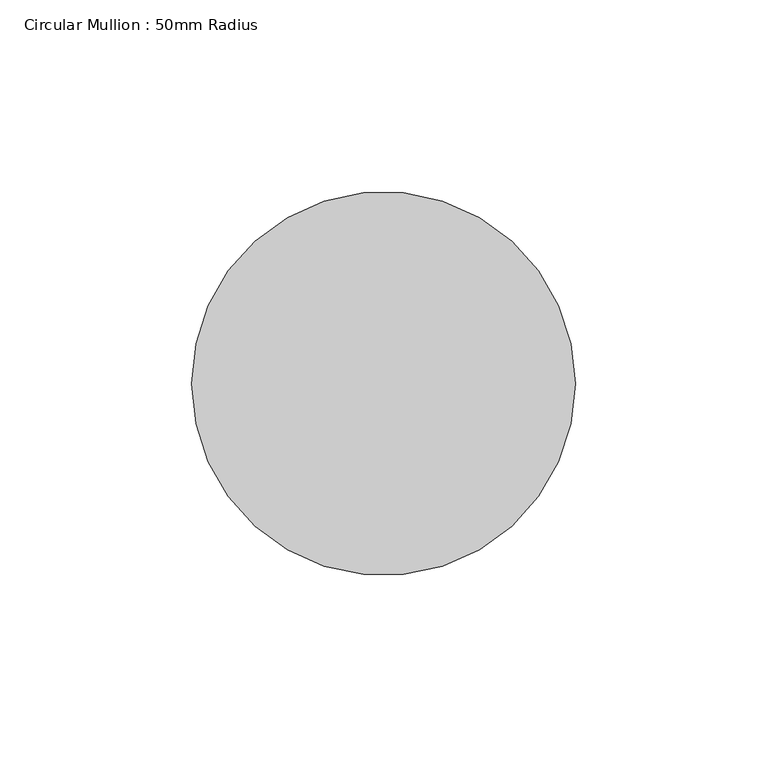
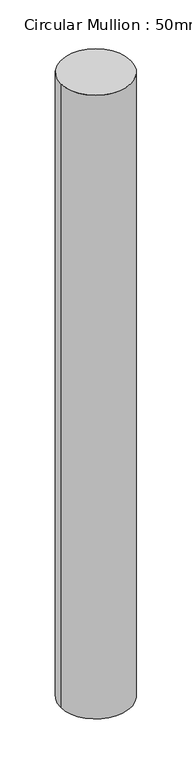
"""IFC4 building model written with IfcOpenShell, lengths in millimetres: member geometry, Circular Mullion : 50mm Radius."""

from ifc_helpers import new_model, si_unit, point, frame, origin, origin_2d, place, context, project, spatial, circle_curve, trimmed, segment, composite_curve, outline, extrude, source, transform, mapped, element, save


def circular_mullion_50mm_radius_1fd985b8(model_context):
    return source(origin(), model_context, "Body", "SweptSolid", [
        extrude(outline(composite_curve([segment(trimmed(circle_curve(origin_2d(), 50.0), [point((50.0, 0.0))], [point((-50.0, 0.0))], False, "CARTESIAN"), True, "CONTINUOUS"), segment(trimmed(circle_curve(origin_2d(), 50.0), [point((-50.0, 0.0))], [point((50.0, 0.0))], False, "CARTESIAN"), True, "CONTINUOUS")], self_intersect=False)), frame((0.0, 0.0, -940.4338252), z_axis=(0.0, 0.0, 1.0), x_axis=(1.0, 0.0, 0.0)), (0.0, 0.0, 1.0), 940.4338252),
    ])


if __name__ == "__main__":
    model = new_model("IFC4")
    model_context = context("Model", 3, world=origin())
    ifc_project = project(units=[si_unit("LENGTHUNIT", "METRE", prefix="MILLI")], contexts=[model_context])
    site = spatial("IfcSite", under=ifc_project)
    building = spatial("IfcBuilding", under=site)
    placement = place(None, origin())
    circular_mullion_50mm_radius_shape = circular_mullion_50mm_radius_1fd985b8(model_context)
    element("IfcMember", 1, ObjectType="Circular Mullion : 50mm Radius", at=placement, inside=building, context=model_context, shape_type="MappedRepresentation", body=[
        mapped(circular_mullion_50mm_radius_shape, transform((0.0, 0.0, 0.0), x_axis=(1.0, 0.0, 0.0), y_axis=(0.0, 1.0, 0.0), z_axis=(0.0, 0.0, 1.0))),
    ])
    save(model, "model.ifc")

# Revit data of these elements
# Type "Circular Mullion : 50mm Radius"
#   built-in parameter 1007350 = 0.164042 (stored number, unit not read)
# Element 1 (IfcMember, "Circular Mullion : 50mm Radius")
#   Materials on its faces: "Aluminium"
# Materials
#   "Aluminium": class "Metal", colour RGB 247 247 247, transparency 0, Description = "Aluminium 6061", Cost = 0
